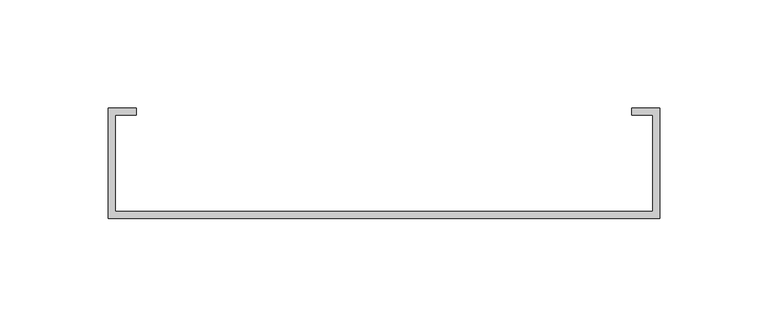
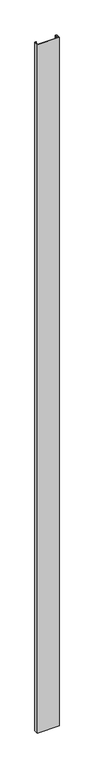
"""IFC4 building model written with IfcOpenShell, lengths in millimetres: proxy geometry, Generic Models 2:Generic Models 2:310765:Generic Models 2:310765 : Generic Models 2:Generic Models 2:310765:1 : Generic Models 2:Generic Models 2:310765:Generic Models 2:310765 : Generic Models 2:Generic Models 2:310765:300385."""

from ifc_helpers import new_model, si_unit, origin, origin_with_axes, place, context, project, spatial, polyline, outline, extrude, source, transform, mapped, element, save


def generic_models_edf6c494(model_context):
    return source(origin(), model_context, "Body", "SweptSolid", [
        extrude(outline(polyline([(667293.3117239, -564707.4790363), (667293.3117239, -564656.6790363), (667306.0117239, -564656.6790363), (667306.0117239, -564659.8540363), (667296.4867239, -564659.8540363), (667296.4867239, -564704.3040363), (667544.1367239, -564704.3040363), (667544.1367239, -564659.8540363), (667534.6117239, -564659.8540363), (667534.6117239, -564656.6790363), (667547.3117239, -564656.6790363), (667547.3117239, -564707.4790363), (667293.3117239, -564707.4790363)])), origin_with_axes(), (0.0, 0.0, 1.0), 8555.7679991),
    ])


if __name__ == "__main__":
    model = new_model("IFC4")
    model_context = context("Model", 3, world=origin())
    ifc_project = project(units=[si_unit("LENGTHUNIT", "METRE", prefix="MILLI")], contexts=[model_context])
    site = spatial("IfcSite", under=ifc_project)
    building = spatial("IfcBuilding", under=site)
    placement = place(None, origin())
    generic_models_shape = generic_models_edf6c494(model_context)
    element("IfcBuildingElementProxy", 1, Name="Generic Models 2:Generic Models 2:310765:Generic Models 2:310765 : Generic Models 2:Generic Models 2:310765:1 : Generic Models 2:Generic Models 2:310765:Generic Models 2:310765 : Generic Models 2:Generic Models 2:310765:300385", ObjectType="Generic Models 2:Generic Models 2:310765:Generic Models 2:310765 : Generic Models 2:Generic Models 2:310765:1 : Generic Models 2:Generic Models 2:310765:Generic Models 2:310765 : Generic Models 2:Generic Models 2:310765:300385", at=placement, inside=building, context=model_context, shape_type="MappedRepresentation", body=[
        mapped(generic_models_shape, transform((0.0, 0.0, 0.0), x_axis=(1.0, 0.0, 0.0), y_axis=(0.0, 1.0, 0.0), z_axis=(0.0, 0.0, 1.0))),
    ])
    save(model, "model.ifc")

# Revit data of these elements
# Type "Generic Models 2:Generic Models 2:310765:Generic Models 2:310765 : Generic Models 2:Generic Models 2:310765:1 : Generic Models 2:Generic Models 2:310765:Generic Models 2:310765 : Generic Models 2:Generic Models 2:310765:300385"
#   NameOverride = "Generic Models 2:Generic Models 2:310765:Generic Models 2:310765 : Generic Models 2:Generic Models 2:310765:300385"
#   ObjectTypeOverride = "Generic Models 2:310765 : Generic Models 2:Generic Models 2:310765"
#   Reference = "Generic Models 2"
#   Tag = "300385"
# Element 1 (IfcBuildingElementProxy, "Generic Models 2:Generic Models 2:310765:Generic Models 2:310765 : Generic Models 2:Generic Models 2:310765:1 : Generic Models 2:Generic Models 2:310765:Generic Models 2:310765 : Generic Models 2:Generic Models 2:310765:300385")
#   Materials on its faces: "STRUCTURAL STEEL - SEE STRUCT. DWGS"
# Materials
#   "STRUCTURAL STEEL - SEE STRUCT. DWGS": class "Metal", colour RGB 189 187 185, transparency 0, Description = "Structural steel 50ksi", Cost = 0
